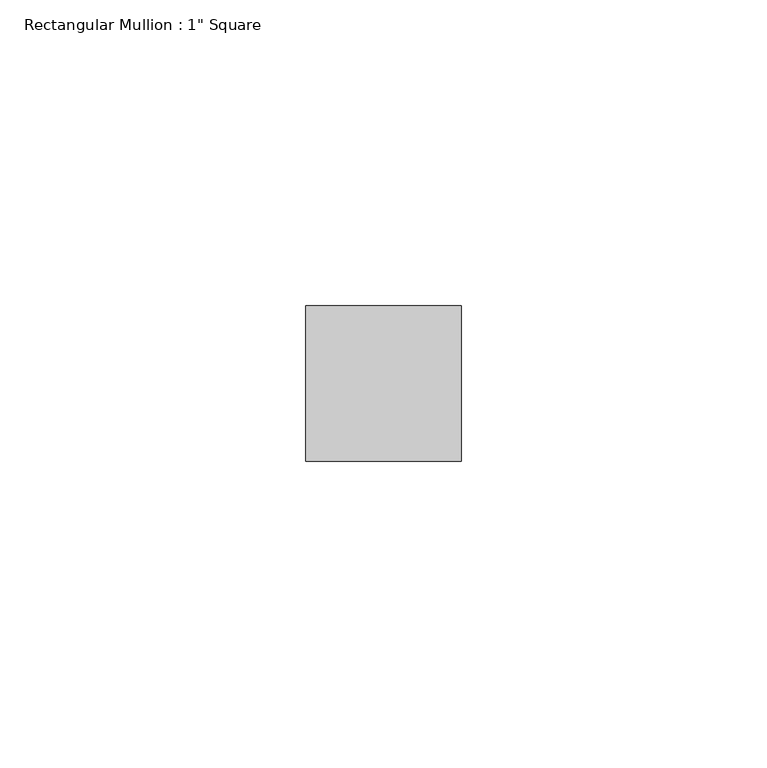
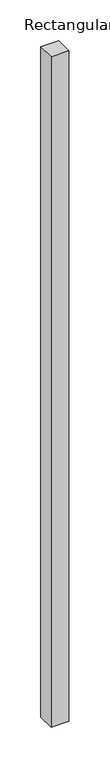
"""IFC4 building model written with IfcOpenShell, lengths in millimetres: member geometry."""

from ifc_helpers import new_model, si_unit, frame, origin, place, context, project, spatial, polyline, outline, extrude, source, transform, mapped, element, save


def member_b874cca0(model_context):
    return source(origin(), model_context, "Body", "SweptSolid", [
        extrude(outline(polyline([(12.7, 12.7), (12.7, -12.7), (-12.7, -12.7), (-12.7, 12.7), (12.7, 12.7)])), frame((0.0, 0.0, -1004.9287927), z_axis=(0.0, 0.0, 1.0), x_axis=(1.0, 0.0, 0.0)), (0.0, 0.0, 1.0), 1004.9287927),
    ])


if __name__ == "__main__":
    model = new_model("IFC4")
    model_context = context("Model", 3, world=origin())
    ifc_project = project(units=[si_unit("LENGTHUNIT", "METRE", prefix="MILLI")], contexts=[model_context])
    site = spatial("IfcSite", under=ifc_project)
    building = spatial("IfcBuilding", under=site)
    placement = place(None, origin())
    member_shape = member_b874cca0(model_context)
    element("IfcMember", 1, ObjectType="Rectangular Mullion : 1\" Square", at=placement, inside=building, context=model_context, shape_type="MappedRepresentation", body=[
        mapped(member_shape, transform((0.0, 0.0, 0.0), x_axis=(1.0, 0.0, 0.0), y_axis=(0.0, 1.0, 0.0), z_axis=(0.0, 0.0, 1.0))),
    ])
    save(model, "model.ifc")

# Revit data of these elements
# Type "Rectangular Mullion : 1\" Square"
#   built-in parameter 1007304 = 0.0833333 (stored number, unit not read)
#   built-in parameter 1007301 = 0.0416667 (stored number, unit not read)
#   built-in parameter 1007300 = 0.0416667 (stored number, unit not read)
# Element 1 (IfcMember, "Rectangular Mullion : 1\" Square")
#   Materials on its faces: "Metal - Aluminum"
# Materials
#   "Metal - Aluminum": class "Metal", colour RGB 247 247 247, transparency 0
